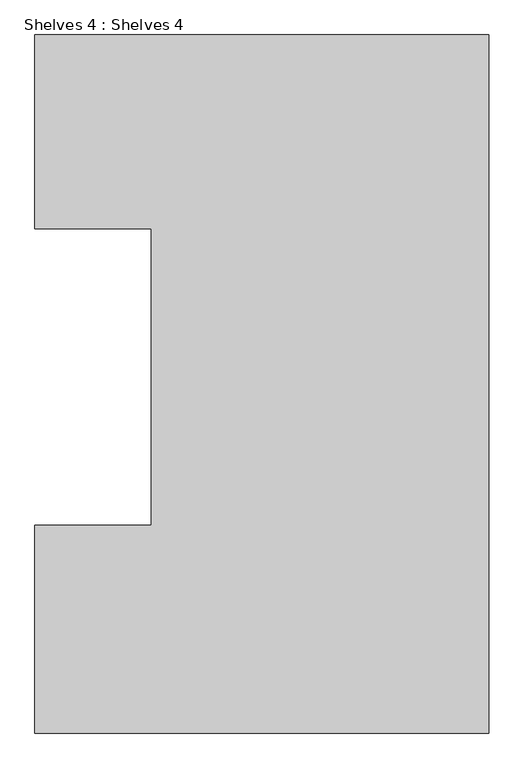
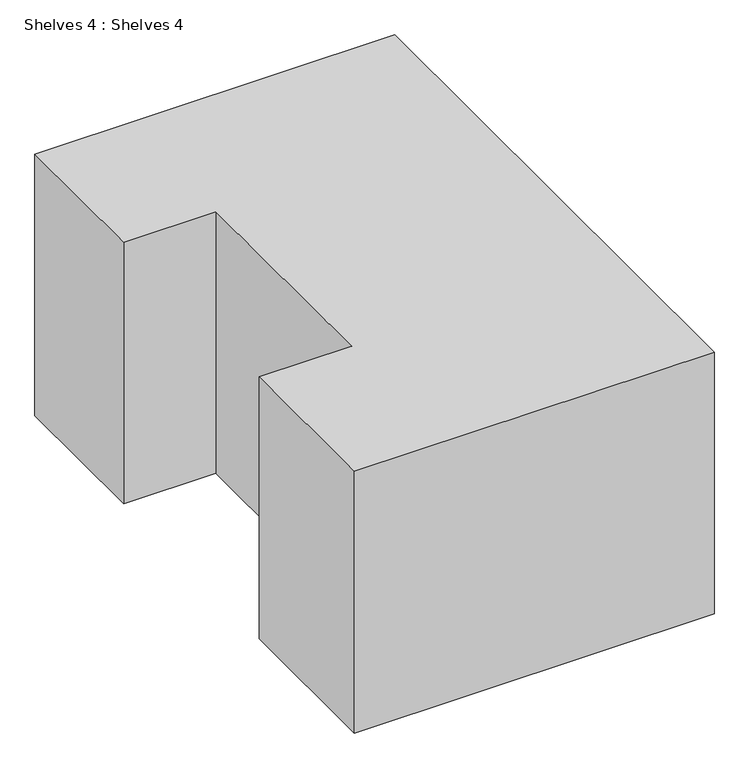
"""IFC4 building model written with IfcOpenShell, lengths in millimetres: furniture geometry, Shelves 4 : Shelves 4."""

from ifc_helpers import new_model, si_unit, origin, origin_with_axes, place, context, project, spatial, polyline, outline, extrude, source, transform, mapped, element, save


def shelves_4_shelves_4_1b616254(model_context):
    return source(origin(), model_context, "Body", "SweptSolid", [
        extrude(outline(polyline([(11900.6870052, 8606.3270218), (11900.6870052, 5558.3270218), (9919.4870052, 5558.3270218), (9919.4870052, 6465.5615366), (10427.4870052, 6465.5615366), (10427.4870052, 7760.9615366), (9919.4870052, 7760.9615366), (9919.4870052, 8606.3270218), (11900.6870052, 8606.3270218)])), origin_with_axes(), (0.0, 0.0, 1.0), 1524.0),
    ])


if __name__ == "__main__":
    model = new_model("IFC4")
    model_context = context("Model", 3, world=origin())
    ifc_project = project(units=[si_unit("LENGTHUNIT", "METRE", prefix="MILLI")], contexts=[model_context])
    site = spatial("IfcSite", under=ifc_project)
    building = spatial("IfcBuilding", under=site)
    placement = place(None, origin())
    shelves_4_shelves_4_shape = shelves_4_shelves_4_1b616254(model_context)
    element("IfcFurniture", 1, ObjectType="Shelves 4 : Shelves 4", at=placement, inside=building, context=model_context, shape_type="MappedRepresentation", body=[
        mapped(shelves_4_shelves_4_shape, transform((0.0, 0.0, 0.0), x_axis=(1.0, 0.0, 0.0), y_axis=(0.0, 1.0, 0.0), z_axis=(0.0, 0.0, 1.0))),
    ])
    save(model, "model.ifc")

# Revit data of these elements
# Element 1 (IfcFurniture, "Shelves 4 : Shelves 4")
#   Materials on its faces: "food"
# Materials
#   "food": class "Glass", colour RGB 233 233 233, transparency 0, Description = "Soda Lime Glass", Cost = 0
